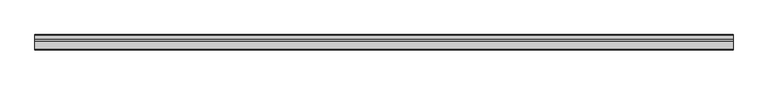
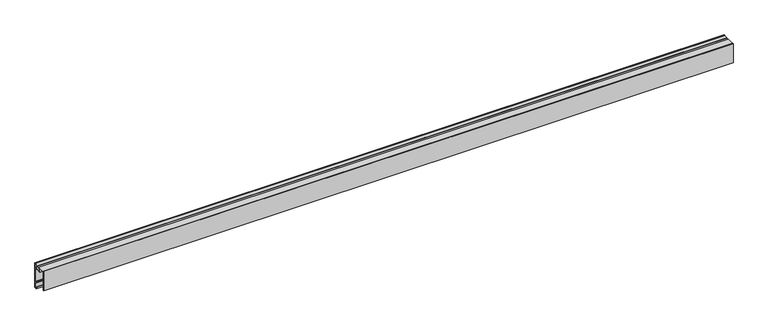
"""IFC4 building model written with IfcOpenShell, lengths in millimetres: proxy geometry, Generic Models 6:Generic Models 2:318829:Generic Models 2:318829 : Generic Models 6:Generic Models 2:318829:3 : Generic Models 6:Generic Models 2:318829:Generic Models 2:318829 : Generic Models 6:Generic Models 2:318829:300683."""

from ifc_helpers import new_model, si_unit, frame, origin, place, context, project, spatial, polyline, outline, extrude, source, transform, mapped, element, save


def generic_models_257d3265(model_context):
    return source(origin(), model_context, "Body", "SweptSolid", [
        extrude(outline(polyline([(-568223.284754, 8552.275728), (-568206.7324978, 8552.275728), (-568206.7324978, 8547.5782294), (-568208.6579133, 8547.5782294), (-568208.6579133, 8545.1969794), (-568206.7324978, 8545.1969794), (-568206.7324978, 8540.4994808), (-568223.284754, 8540.4994808), (-568223.284754, 8545.1969794), (-568221.3593386, 8545.1969794), (-568221.3593386, 8547.5782294), (-568223.284754, 8547.5782294), (-568223.284754, 8552.275728)])), frame((591391.6367242, 0.0, 0.0), z_axis=(1.0, 0.0, 0.0), x_axis=(0.0, 1.0, 0.0)), (0.0, 0.0, 1.0), 2438.4),
        extrude(outline(polyline([(-568196.8049878, 8554.260103), (-568196.8049878, 8555.847603), (-568195.2174878, 8555.847603), (-568195.2174878, 8463.847603), (-568203.6638594, 8463.847603), (-568203.6638594, 8468.2349296), (-568202.0763594, 8468.2349296), (-568202.0763594, 8465.435103), (-568196.8049878, 8465.435103), (-568196.8049878, 8485.435103), (-568203.6638594, 8485.435103), (-568203.6638594, 8489.8224296), (-568202.0763594, 8489.8224296), (-568202.0763594, 8487.022603), (-568196.8049878, 8487.022603), (-568196.8049878, 8538.5151058), (-568210.5028103, 8538.5151058), (-568210.5028103, 8540.1026058), (-568206.3356228, 8540.1026058), (-568206.3356228, 8545.5938544), (-568208.2610383, 8545.5938544), (-568208.2610383, 8547.1813544), (-568206.3356228, 8547.1813544), (-568206.3356228, 8552.672603), (-568210.5028103, 8552.672603), (-568210.5028103, 8554.260103), (-568196.8049878, 8554.260103)]), holes=[polyline([(-568196.8049878, 8540.1026058), (-568196.8049878, 8552.672603), (-568204.7481228, 8552.672603), (-568204.7481228, 8540.1026058), (-568196.8049878, 8540.1026058)])]), frame((591391.6367242, 0.0, 0.0), z_axis=(1.0, 0.0, 0.0), x_axis=(0.0, 1.0, 0.0)), (0.0, 0.0, 1.0), 2438.4),
        extrude(outline(polyline([(-568246.5023979, 8485.435103), (-568246.5023979, 8483.847603), (-568249.2174878, 8483.847603), (-568249.2174878, 8555.847603), (-568247.6299878, 8555.847603), (-568247.6299878, 8554.260103), (-568219.5144415, 8554.260103), (-568219.5144415, 8552.672603), (-568223.681629, 8552.672603), (-568223.681629, 8547.1813544), (-568221.7562136, 8547.1813544), (-568221.7562136, 8545.5938544), (-568223.681629, 8545.5938544), (-568223.681629, 8540.1026058), (-568219.5144415, 8540.1026058), (-568219.5144415, 8538.5151058), (-568225.269129, 8538.5151058), (-568225.269129, 8552.672603), (-568247.6299878, 8552.672603), (-568247.6299878, 8485.435103), (-568246.5023979, 8485.435103)])), frame((591391.6367242, 0.0, 0.0), z_axis=(1.0, 0.0, 0.0), x_axis=(0.0, 1.0, 0.0)), (0.0, 0.0, 1.0), 2438.4),
    ])


if __name__ == "__main__":
    model = new_model("IFC4")
    model_context = context("Model", 3, world=origin())
    ifc_project = project(units=[si_unit("LENGTHUNIT", "METRE", prefix="MILLI")], contexts=[model_context])
    site = spatial("IfcSite", under=ifc_project)
    building = spatial("IfcBuilding", under=site)
    placement = place(None, origin())
    generic_models_shape = generic_models_257d3265(model_context)
    element("IfcBuildingElementProxy", 1, Name="Generic Models 6:Generic Models 2:318829:Generic Models 2:318829 : Generic Models 6:Generic Models 2:318829:3 : Generic Models 6:Generic Models 2:318829:Generic Models 2:318829 : Generic Models 6:Generic Models 2:318829:300683", ObjectType="Generic Models 6:Generic Models 2:318829:Generic Models 2:318829 : Generic Models 6:Generic Models 2:318829:3 : Generic Models 6:Generic Models 2:318829:Generic Models 2:318829 : Generic Models 6:Generic Models 2:318829:300683", at=placement, inside=building, context=model_context, shape_type="MappedRepresentation", body=[
        mapped(generic_models_shape, transform((0.0, 0.0, 0.0), x_axis=(1.0, 0.0, 0.0), y_axis=(0.0, 1.0, 0.0), z_axis=(0.0, 0.0, 1.0))),
    ])
    save(model, "model.ifc")

# Revit data of these elements
# Type "Generic Models 6:Generic Models 2:318829:Generic Models 2:318829 : Generic Models 6:Generic Models 2:318829:3 : Generic Models 6:Generic Models 2:318829:Generic Models 2:318829 : Generic Models 6:Generic Models 2:318829:300683"
#   NameOverride = "Generic Models 6:Generic Models 2:318829:Generic Models 2:318829 : Generic Models 6:Generic Models 2:318829:300683"
#   ObjectTypeOverride = "Generic Models 2:318829 : Generic Models 6:Generic Models 2:318829"
#   Reference = "Generic Models 2"
#   Tag = "300683"
# Element 1 (IfcBuildingElementProxy, "Generic Models 6:Generic Models 2:318829:Generic Models 2:318829 : Generic Models 6:Generic Models 2:318829:3 : Generic Models 6:Generic Models 2:318829:Generic Models 2:318829 : Generic Models 6:Generic Models 2:318829:300683")
#   Materials on its faces: "THERMAL BROKEN ALUMINUM STOREFRONT FOR POLYCARBONATE"
# Materials
#   "THERMAL BROKEN ALUMINUM STOREFRONT FOR POLYCARBONATE": class "Unassigned", colour RGB 244 244 244, transparency 0, Keynote = "M07611300.01", Cost = 0
